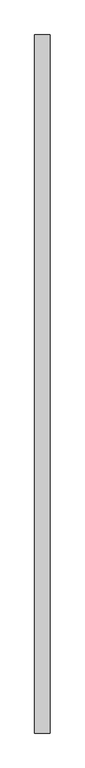
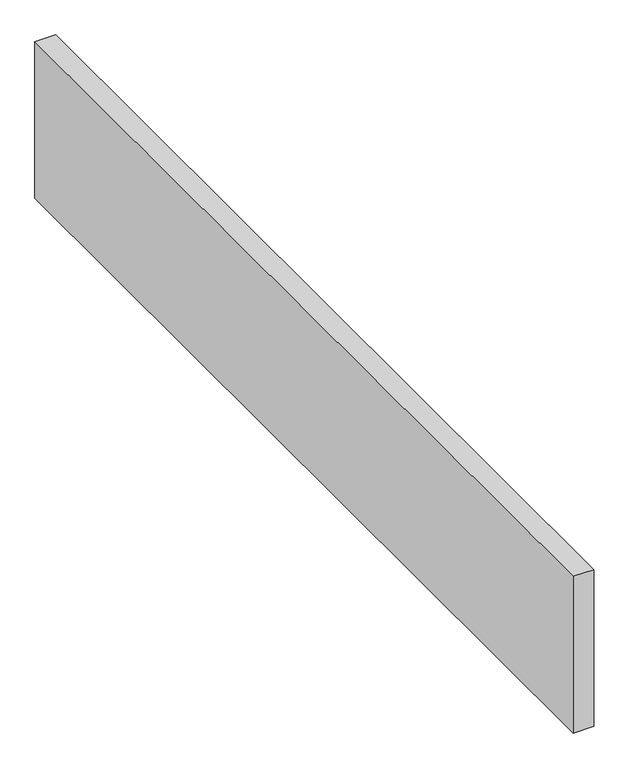
"""IFC4 building model written with IfcOpenShell, lengths in millimetres: proxy geometry, Framing059 2618 : Framing059 2618."""

from ifc_helpers import new_model, si_unit, frame, origin, place, context, project, spatial, polyline, outline, extrude, source, transform, mapped, element, save


def generic_models_e6aee20f(model_context):
    return source(origin(), model_context, "Body", "SweptSolid", [
        extrude(outline(polyline([(-2199.7519086, -1052.8906574), (-2244.2019086, -1052.8906574), (-2244.2019086, 947.1093426), (-2199.7519086, 947.1093426), (-2199.7519086, -1052.8906574)])), frame((0.0, 0.0, 42134.105552), z_axis=(0.0, 0.0, 1.0), x_axis=(1.0, 0.0, 0.0)), (0.0, 0.0, 1.0), 355.2981173),
    ])


if __name__ == "__main__":
    model = new_model("IFC4")
    model_context = context("Model", 3, world=origin())
    ifc_project = project(units=[si_unit("LENGTHUNIT", "METRE", prefix="MILLI")], contexts=[model_context])
    site = spatial("IfcSite", under=ifc_project)
    building = spatial("IfcBuilding", under=site)
    placement = place(None, origin())
    generic_models_shape = generic_models_e6aee20f(model_context)
    element("IfcBuildingElementProxy", 1, Name="Framing059 2618 : Framing059 2618", ObjectType="Framing059 2618 : Framing059 2618", at=placement, inside=building, context=model_context, shape_type="MappedRepresentation", body=[
        mapped(generic_models_shape, transform((0.0, 0.0, 0.0), x_axis=(1.0, 0.0, 0.0), y_axis=(0.0, 1.0, 0.0), z_axis=(0.0, 0.0, 1.0))),
    ])
    save(model, "model.ifc")

# Revit data of these elements
# Type "Framing059 2618 : Framing059 2618"
#   NameOverride = "Framing059"
# Element 1 (IfcBuildingElementProxy, "Framing059 2618 : Framing059 2618")
#   Materials on its faces: "WOOD FRAMING (SEE STRUCT DWGS)"
# Materials
#   "WOOD FRAMING (SEE STRUCT DWGS)": class "Unassigned", colour RGB 224 188 168, transparency 0, Cost = 0
